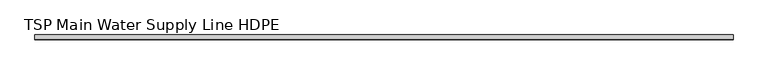
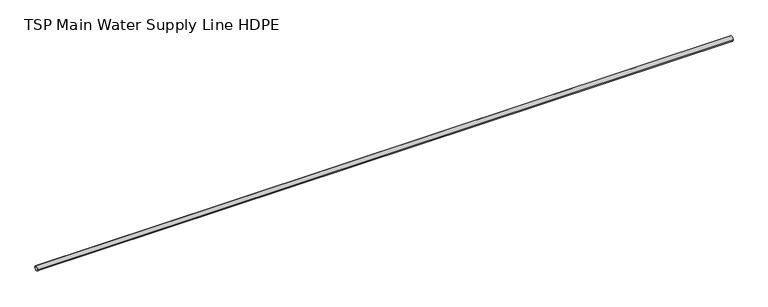
"""IFC4 building model written with IfcOpenShell, lengths in millimetres: flow terminal geometry, TSP Main Water Supply Line HDPE : HDPE Fresh Water Supply."""

from ifc_helpers import new_model, si_unit, point, frame, origin, origin_2d, place, context, project, spatial, circle_curve, trimmed, segment, composite_curve, outline, extrude, source, transform, mapped, element, save


def tsp_main_water_supply_line_hdpe_931aad72(model_context):
    return source(origin(), model_context, "Body", "SweptSolid", [
        extrude(outline(composite_curve([segment(trimmed(circle_curve(origin_2d(), 16.0), [point((-16.0, 0.0))], [point((16.0, 0.0))], False, "CARTESIAN"), True, "CONTINUOUS"), segment(trimmed(circle_curve(origin_2d(), 16.0), [point((16.0, 0.0))], [point((-16.0, 0.0))], False, "CARTESIAN"), True, "CONTINUOUS")], self_intersect=False), holes=[composite_curve([segment(trimmed(circle_curve(origin_2d(), 15.0), [point((-15.0, 0.0))], [point((15.0, 0.0))], True, "CARTESIAN"), True, "CONTINUOUS"), segment(trimmed(circle_curve(origin_2d(), 15.0), [point((15.0, 0.0))], [point((-15.0, 0.0))], True, "CARTESIAN"), True, "CONTINUOUS")], self_intersect=False)]), frame((0.0, 0.0, 0.0), z_axis=(1.0, 0.0, 0.0), x_axis=(0.0, 1.0, 0.0)), (0.0, 0.0, 1.0), 4676.3984473),
    ])


if __name__ == "__main__":
    model = new_model("IFC4")
    model_context = context("Model", 3, world=origin())
    ifc_project = project(units=[si_unit("LENGTHUNIT", "METRE", prefix="MILLI")], contexts=[model_context])
    site = spatial("IfcSite", under=ifc_project)
    building = spatial("IfcBuilding", under=site)
    placement = place(None, origin())
    tsp_main_water_supply_line_hdpe_shape = tsp_main_water_supply_line_hdpe_931aad72(model_context)
    element("IfcFlowTerminal", 1, ObjectType="TSP Main Water Supply Line HDPE : HDPE Fresh Water Supply", at=placement, inside=building, context=model_context, shape_type="MappedRepresentation", body=[
        mapped(tsp_main_water_supply_line_hdpe_shape, transform((0.0, 0.0, 0.0), x_axis=(1.0, 0.0, 0.0), y_axis=(0.0, 1.0, 0.0), z_axis=(0.0, 0.0, 1.0))),
    ])
    save(model, "model.ifc")

# Revit data of these elements
# Type "TSP Main Water Supply Line HDPE : HDPE Fresh Water Supply"
#   Model = "TSP_110SFWSP"
#   Pipe length [instance default] = 1200 mm
#   Pipe dia = 30 mm
#   built-in parameter 1001306 [instance default] = 3.93701 (stored number, unit not read)
#   Default Elevation = 0
# Element 1 (IfcFlowTerminal, "TSP Main Water Supply Line HDPE : HDPE Fresh Water Supply")
#   Pipe length = 4676.398 mm
#   built-in parameter 1001306 = 15.3425 (stored number, unit not read)
#   Materials on its faces: "Aluminum, Anodized Blue"
# Materials
#   "Aluminum, Anodized Blue": class "Metal", colour RGB 120 120 120, transparency 0, Description = "Anodized aluminum, blue", Cost = 0
